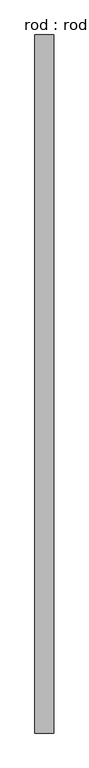
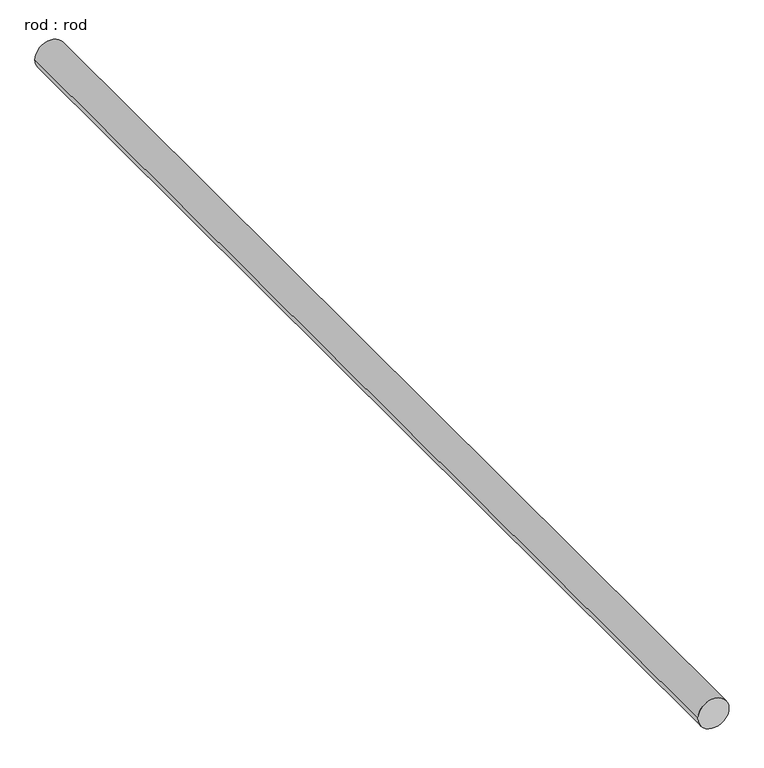
"""IFC4 building model written with IfcOpenShell, lengths in millimetres: proxy geometry, rod : rod."""

from ifc_helpers import new_model, si_unit, point, frame, frame_2d, origin, place, context, project, spatial, circle_curve, trimmed, segment, composite_curve, outline, extrude, source, transform, mapped, element, save


def rod_rod_3c23be87(model_context):
    return source(origin(), model_context, "Body", "SweptSolid", [
        extrude(outline(composite_curve([segment(trimmed(circle_curve(frame_2d((0.0108462, 0.0)), 200.0), [point((0.0108462, 200.0))], [point((0.0108462, -200.0))], False, "CARTESIAN"), True, "CONTINUOUS"), segment(trimmed(circle_curve(frame_2d((0.0108462, 0.0)), 200.0), [point((0.0108462, -200.0))], [point((0.0108462, 200.0))], False, "CARTESIAN"), True, "CONTINUOUS")], self_intersect=False)), frame((0.0, -3326.9142418, 0.0), z_axis=(0.0, 1.0, 0.0), x_axis=(0.0, 0.0, 1.0)), (0.0, 0.0, 1.0), 14839.2857143),
    ])


if __name__ == "__main__":
    model = new_model("IFC4")
    model_context = context("Model", 3, world=origin())
    ifc_project = project(units=[si_unit("LENGTHUNIT", "METRE", prefix="MILLI")], contexts=[model_context])
    site = spatial("IfcSite", under=ifc_project)
    building = spatial("IfcBuilding", under=site)
    placement = place(None, origin())
    rod_rod_shape = rod_rod_3c23be87(model_context)
    element("IfcBuildingElementProxy", 1, Name="rod : rod", ObjectType="rod : rod", at=placement, inside=building, context=model_context, shape_type="MappedRepresentation", body=[
        mapped(rod_rod_shape, transform((0.0, 0.0, 0.0), x_axis=(1.0, 0.0, 0.0), y_axis=(0.0, 1.0, 0.0), z_axis=(0.0, 0.0, 1.0))),
    ])
    save(model, "model.ifc")

# Revit data of these elements
# Type "rod : rod"
#   Default Elevation = 0
